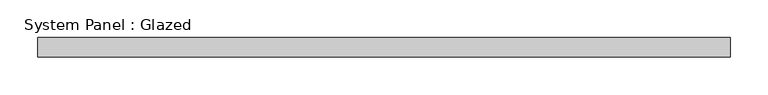
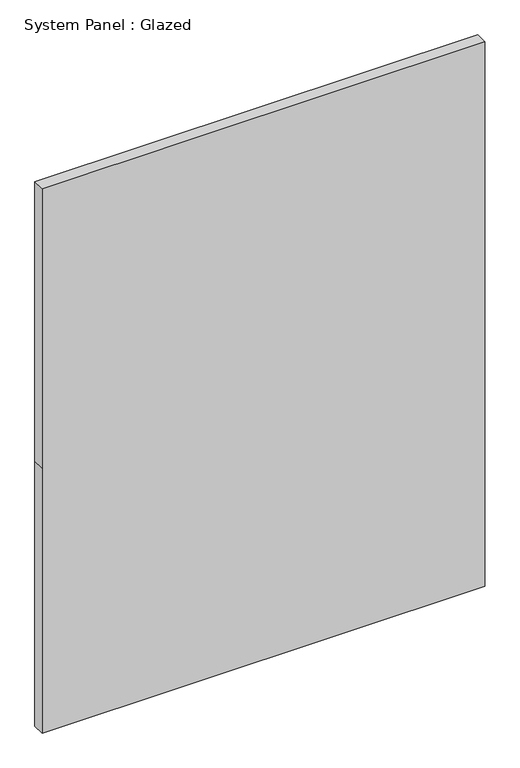
"""IFC4 building model written with IfcOpenShell, lengths in millimetres: plate geometry, System Panel : Glazed."""

import ifcopenshell
import ifcopenshell.guid

model = None  # the IFC model being written
_history = None  # IfcOwnerHistory: only IFC2X3 demands one
_inside = {}  # id of a spatial element -> (the spatial element, [elements in it])
_under = {}  # id of a project, library or spatial element -> (it, [spatial elements below it])
_declared = {}  # id of a project -> (the project, [libraries it declares])
_typed = {}  # id of a type object -> (the type object, [elements of that type])
_made_of = {}  # id of a material, layer set ... -> (it, [elements and type objects made of it])


def new_model(schema):
    """Start an empty IFC model of exactly this schema.

    Asked for "IFC4X3", IfcOpenShell would pick the latest addendum, in which some entities
    have other attributes; the version numbers below select the first issue.
    IFC2X3 requires an IfcOwnerHistory on every rooted entity: one is made here for all.
    """
    global model, _history
    if schema == "IFC4X3":
        model = ifcopenshell.file(schema_version=(4, 3, 0, 0))
    else:
        model = ifcopenshell.file(schema=schema)
    _inside.clear()
    _under.clear()
    _declared.clear()
    _typed.clear()
    _made_of.clear()
    _history = None
    if model.schema == "IFC2X3":
        org = make("IfcOrganization", Name="unknown")
        user = make(
            "IfcPersonAndOrganization",
            ThePerson=make("IfcPerson", FamilyName="unknown"),
            TheOrganization=org,
        )
        app = make(
            "IfcApplication",
            ApplicationDeveloper=org,
            Version="unknown",
            ApplicationFullName="unknown",
            ApplicationIdentifier="unknown",
        )
        _history = make(
            "IfcOwnerHistory",
            OwningUser=user,
            OwningApplication=app,
            ChangeAction="ADDED",
            CreationDate=0,
        )
    return model


def make(cls, **values):
    """One entity of the class cls with the attributes given. An attribute that is None is left unset."""
    return model.create_entity(
        cls, **{name: value for name, value in values.items() if value is not None}
    )


def rooted(cls, **values):
    """An entity with a GlobalId (a new one), such as an element, a storey or a relation."""
    return make(cls, GlobalId=ifcopenshell.guid.new(), OwnerHistory=_history, **values)


def si_unit(unit_type, name, prefix=None):
    """IfcSIUnit, for example si_unit("LENGTHUNIT", "METRE", prefix="MILLI")."""
    return make("IfcSIUnit", UnitType=unit_type, Prefix=prefix, Name=name)


def assignment(units):
    """IfcUnitAssignment: the units of a project."""
    return None if units is None else make("IfcUnitAssignment", Units=units)


def point(xyz):
    """IfcCartesianPoint."""
    return None if xyz is None else make("IfcCartesianPoint", Coordinates=xyz)


def direction(xyz):
    """IfcDirection."""
    return None if xyz is None else make("IfcDirection", DirectionRatios=xyz)


def frame(location, z_axis=None, x_axis=None):
    """IfcAxis2Placement3D, a coordinate frame: its origin and axes. An axis left out is left unset."""
    return make(
        "IfcAxis2Placement3D",
        Location=point(location),
        Axis=direction(z_axis),
        RefDirection=direction(x_axis),
    )


def origin():
    """The frame at (0, 0, 0) with its axes left unset."""
    return frame((0.0, 0.0, 0.0))


def place(relative_to, where):
    """IfcLocalPlacement: puts the frame where relative to a parent placement (None: the world)."""
    return make(
        "IfcLocalPlacement", PlacementRelTo=relative_to, RelativePlacement=where
    )


def context(
    kind, dimensions, precision=None, world=None, true_north=None, identifier=None
):
    """IfcGeometricRepresentationContext, for example the 3D "Model" context."""
    return make(
        "IfcGeometricRepresentationContext",
        ContextIdentifier=identifier,
        ContextType=kind,
        CoordinateSpaceDimension=dimensions,
        Precision=precision,
        WorldCoordinateSystem=world,
        TrueNorth=true_north,
    )


def project(units=None, contexts=None):
    """IfcProject with its units and contexts."""
    return rooted(
        "IfcProject",
        Name="project",
        RepresentationContexts=contexts,
        UnitsInContext=assignment(units),
    )


def spatial(cls, under=None, at=None, **own):
    """A site, building, storey or space (cls), placed at a placement, below another one or the project."""
    s = rooted(cls, ObjectPlacement=at, **own)
    if under is not None:
        _under.setdefault(under.id(), (under, []))[1].append(s)
    return s


def polyline(points):
    """IfcPolyline through the points."""
    return make("IfcPolyline", Points=[point(p) for p in points])


def outline(outer, holes=None, kind="AREA"):
    """IfcArbitraryClosedProfileDef: a profile drawn as a closed curve; with holes, ...WithVoids."""
    if holes is None:
        return make("IfcArbitraryClosedProfileDef", ProfileType=kind, OuterCurve=outer)
    return make(
        "IfcArbitraryProfileDefWithVoids",
        ProfileType=kind,
        OuterCurve=outer,
        InnerCurves=holes,
    )


def extrude(swept, where, along, depth):
    """IfcExtrudedAreaSolid: the profile swept, set in the frame where, extruded along a direction by depth."""
    return make(
        "IfcExtrudedAreaSolid",
        SweptArea=swept,
        Position=where,
        ExtrudedDirection=direction(along),
        Depth=depth,
    )


def shape(context_of_items, identifier, shape_type, items):
    """IfcShapeRepresentation: the items that make up one representation, for example the "Body"."""
    return make(
        "IfcShapeRepresentation",
        ContextOfItems=context_of_items,
        RepresentationIdentifier=identifier,
        RepresentationType=shape_type,
        Items=items,
    )


def source(mapping_origin, context_of_items, identifier, shape_type, items):
    """IfcRepresentationMap: a shape defined once, which mapped items show again and again."""
    return make(
        "IfcRepresentationMap",
        MappingOrigin=mapping_origin,
        MappedRepresentation=shape(context_of_items, identifier, shape_type, items),
    )


def transform(
    local_origin,
    x_axis=None,
    y_axis=None,
    z_axis=None,
    scale=None,
    scale2=None,
    scale3=None,
    uniform=True,
):
    """IfcCartesianTransformationOperator3D, or its non-uniform kind. x_axis, y_axis, z_axis: its Axis1, 2, 3."""
    if uniform:
        return make(
            "IfcCartesianTransformationOperator3D",
            Axis1=direction(x_axis),
            Axis2=direction(y_axis),
            LocalOrigin=point(local_origin),
            Scale=scale,
            Axis3=direction(z_axis),
        )
    return make(
        "IfcCartesianTransformationOperator3DnonUniform",
        Axis1=direction(x_axis),
        Axis2=direction(y_axis),
        LocalOrigin=point(local_origin),
        Scale=scale,
        Axis3=direction(z_axis),
        Scale2=scale2,
        Scale3=scale3,
    )


def mapped(mapping_source, mapping_target):
    """IfcMappedItem: shows the shape of a source again, moved by a transform."""
    return make(
        "IfcMappedItem", MappingSource=mapping_source, MappingTarget=mapping_target
    )


def made_of(thing, what):
    """Note that an element or type object is made of a material, layer set ...; save() writes the relation."""
    if what is not None:
        _made_of.setdefault(what.id(), (what, []))[1].append(thing)
    return thing


def element(
    cls,
    number,
    at=None,
    inside=None,
    cuts=None,
    type_object=None,
    material=None,
    context=None,
    identifier="Body",
    shape_type=None,
    held_by="IfcProductDefinitionShape",
    body=None,
    shapes=None,
    **own,
):
    """One element of the class cls, such as IfcWall. Its Tag is "e" and its number.

    at: its placement. inside: the storey or other place that contains it. cuts: it is an
    opening in that element (IfcRelVoidsElement). A single representation is given by context,
    identifier, shape_type and body (its items); several are given by shapes. held_by: the class
    of the entity that holds the representations. save() writes the other relations.
    """
    e = rooted(cls, Tag="e%d" % number, ObjectPlacement=at, **own)
    if body is not None:
        shapes = [shape(context, identifier, shape_type, body)]
    if shapes is not None:
        e.Representation = make(held_by, Representations=shapes)
    if inside is not None:
        _inside.setdefault(inside.id(), (inside, []))[1].append(e)
    if cuts is not None:
        rooted(
            "IfcRelVoidsElement", RelatingBuildingElement=cuts, RelatedOpeningElement=e
        )
    if type_object is not None:
        _typed.setdefault(type_object.id(), (type_object, []))[1].append(e)
    return made_of(e, material)


def aggregate(whole, parts):
    """IfcRelAggregates: a whole, such as a stair, and the parts it consists of."""
    return rooted("IfcRelAggregates", RelatingObject=whole, RelatedObjects=parts)


def save(model, path):
    """Write the relations noted so far, then the file.

    IfcRelAggregates (storeys below a building ...), IfcRelContainedInSpatialStructure (elements
    in a storey), IfcRelDefinesByType, IfcRelAssociatesMaterial and IfcRelDeclares: one each for
    every whole, place, type object, material and project.
    """
    for whole, parts in _under.values():
        aggregate(whole, parts)
    for where, things in _inside.values():
        rooted(
            "IfcRelContainedInSpatialStructure",
            RelatedElements=things,
            RelatingStructure=where,
        )
    for kind, things in _typed.values():
        rooted("IfcRelDefinesByType", RelatedObjects=things, RelatingType=kind)
    for what, things in _made_of.values():
        rooted("IfcRelAssociatesMaterial", RelatedObjects=things, RelatingMaterial=what)
    for by, libraries in _declared.values():
        rooted("IfcRelDeclares", RelatingContext=by, RelatedDefinitions=libraries)
    model.write(path)


def system_panel_glazed_89462941(model_context):
    return source(origin(), model_context, "Body", "SweptSolid", [
        extrude(outline(polyline([(0.0, -456.6708333), (0.0, 456.6708333), (577.85, 456.6708333), (1187.45, 456.6708333), (1187.45, -456.6708333), (577.85, -456.6708333), (0.0, -456.6708333)])), frame((0.0, -44.45, 0.0), z_axis=(0.0, 1.0, 0.0), x_axis=(0.0, 0.0, 1.0)), (0.0, 0.0, 1.0), 25.4),
    ])


if __name__ == "__main__":
    model = new_model("IFC4")
    model_context = context("Model", 3, world=origin())
    ifc_project = project(units=[si_unit("LENGTHUNIT", "METRE", prefix="MILLI")], contexts=[model_context])
    site = spatial("IfcSite", under=ifc_project)
    building = spatial("IfcBuilding", under=site)
    placement = place(None, origin())
    system_panel_glazed_shape = system_panel_glazed_89462941(model_context)
    element("IfcPlate", 1, ObjectType="System Panel : Glazed", at=placement, inside=building, context=model_context, shape_type="MappedRepresentation", body=[
        mapped(system_panel_glazed_shape, transform((0.0, 0.0, 0.0), x_axis=(1.0, 0.0, 0.0), y_axis=(0.0, 1.0, 0.0), z_axis=(0.0, 0.0, 1.0))),
    ])
    save(model, "model.ifc")

# Revit data of these elements
# Element 1 (IfcPlate, "System Panel : Glazed")
#   Materials on its faces: "Glass"
# Materials
#   "Glass": class "Unassigned", colour RGB 0 0 255, transparency 0.75
